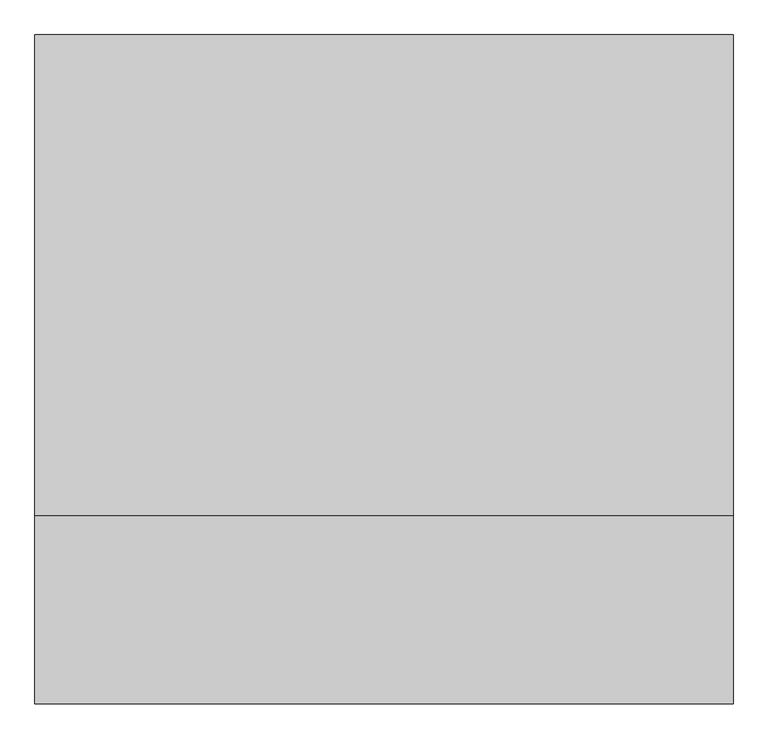
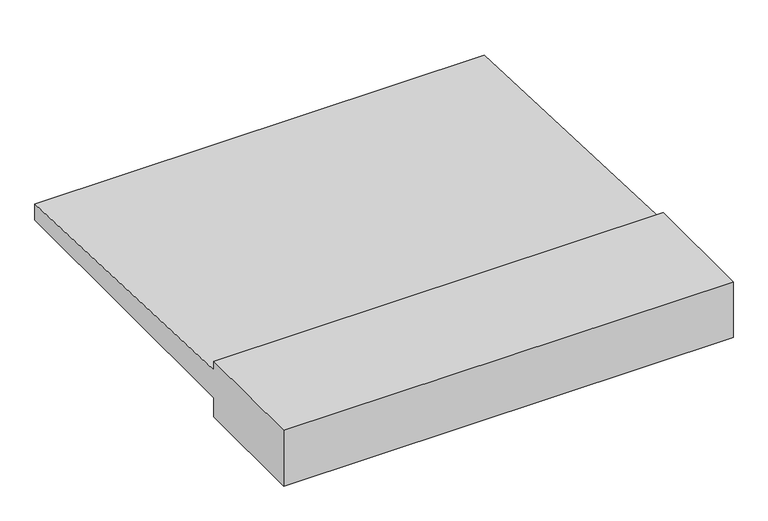
"""IFC4 building model written with IfcOpenShell, lengths in millimetres: plate geometry, 캐노피 : 캐노피."""

from ifc_helpers import new_model, si_unit, frame, origin, place, context, project, spatial, polyline, outline, extrude, source, transform, mapped, element, save


def plate_1abda111(model_context):
    return source(origin(), model_context, "Body", "SweptSolid", [
        extrude(outline(polyline([(-195.0, 800.0), (-195.0, 990.0), (195.0, 990.0), (195.0, 960.0), (1195.0, 920.0), (1195.0, 865.0), (195.0, 865.0), (195.0, 800.0), (-195.0, 800.0)])), frame((-725.0, 0.0, 0.0), z_axis=(1.0, 0.0, 0.0), x_axis=(0.0, 1.0, 0.0)), (0.0, 0.0, 1.0), 1450.0),
    ])


if __name__ == "__main__":
    model = new_model("IFC4")
    model_context = context("Model", 3, world=origin())
    ifc_project = project(units=[si_unit("LENGTHUNIT", "METRE", prefix="MILLI")], contexts=[model_context])
    site = spatial("IfcSite", under=ifc_project)
    building = spatial("IfcBuilding", under=site)
    placement = place(None, origin())
    plate_shape = plate_1abda111(model_context)
    element("IfcPlate", 1, ObjectType="캐노피 : 캐노피", at=placement, inside=building, context=model_context, shape_type="MappedRepresentation", body=[
        mapped(plate_shape, transform((0.0, 0.0, 0.0), x_axis=(1.0, 0.0, 0.0), y_axis=(0.0, 1.0, 0.0), z_axis=(0.0, 0.0, 1.0))),
    ])
    save(model, "model.ifc")

# Revit data of these elements
# Type "캐노피 : 캐노피"
#   Type Mark = "203"
#   Width = 1450 mm
#   Height = 190 mm
#   돌출길이 = 1000 mm
#   Default Sill Height = 800 mm
#   Wall Closure = (empty or 0)
